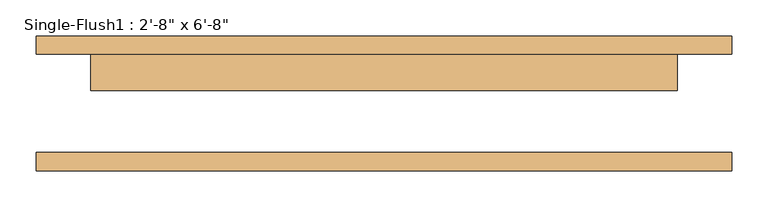
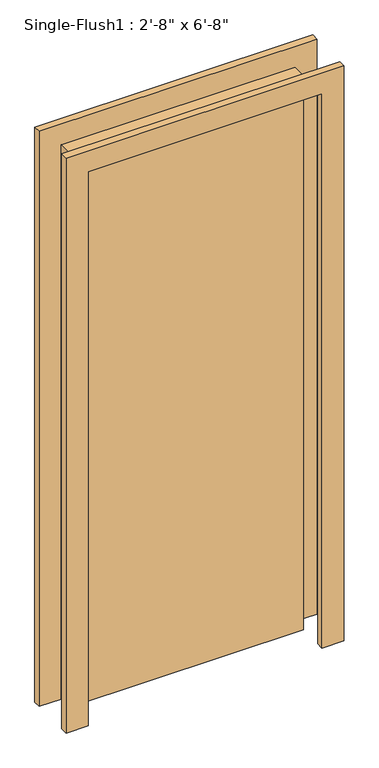
"""IFC4 building model written with IfcOpenShell, lengths in millimetres: door geometry."""

import ifcopenshell
import ifcopenshell.guid

model = None  # the IFC model being written
_history = None  # IfcOwnerHistory: only IFC2X3 demands one
_inside = {}  # id of a spatial element -> (the spatial element, [elements in it])
_under = {}  # id of a project, library or spatial element -> (it, [spatial elements below it])
_declared = {}  # id of a project -> (the project, [libraries it declares])
_typed = {}  # id of a type object -> (the type object, [elements of that type])
_made_of = {}  # id of a material, layer set ... -> (it, [elements and type objects made of it])


def new_model(schema):
    """Start an empty IFC model of exactly this schema.

    Asked for "IFC4X3", IfcOpenShell would pick the latest addendum, in which some entities
    have other attributes; the version numbers below select the first issue.
    IFC2X3 requires an IfcOwnerHistory on every rooted entity: one is made here for all.
    """
    global model, _history
    if schema == "IFC4X3":
        model = ifcopenshell.file(schema_version=(4, 3, 0, 0))
    else:
        model = ifcopenshell.file(schema=schema)
    _inside.clear()
    _under.clear()
    _declared.clear()
    _typed.clear()
    _made_of.clear()
    _history = None
    if model.schema == "IFC2X3":
        org = make("IfcOrganization", Name="unknown")
        user = make(
            "IfcPersonAndOrganization",
            ThePerson=make("IfcPerson", FamilyName="unknown"),
            TheOrganization=org,
        )
        app = make(
            "IfcApplication",
            ApplicationDeveloper=org,
            Version="unknown",
            ApplicationFullName="unknown",
            ApplicationIdentifier="unknown",
        )
        _history = make(
            "IfcOwnerHistory",
            OwningUser=user,
            OwningApplication=app,
            ChangeAction="ADDED",
            CreationDate=0,
        )
    return model


def make(cls, **values):
    """One entity of the class cls with the attributes given. An attribute that is None is left unset."""
    return model.create_entity(
        cls, **{name: value for name, value in values.items() if value is not None}
    )


def rooted(cls, **values):
    """An entity with a GlobalId (a new one), such as an element, a storey or a relation."""
    return make(cls, GlobalId=ifcopenshell.guid.new(), OwnerHistory=_history, **values)


def si_unit(unit_type, name, prefix=None):
    """IfcSIUnit, for example si_unit("LENGTHUNIT", "METRE", prefix="MILLI")."""
    return make("IfcSIUnit", UnitType=unit_type, Prefix=prefix, Name=name)


def assignment(units):
    """IfcUnitAssignment: the units of a project."""
    return None if units is None else make("IfcUnitAssignment", Units=units)


def point(xyz):
    """IfcCartesianPoint."""
    return None if xyz is None else make("IfcCartesianPoint", Coordinates=xyz)


def direction(xyz):
    """IfcDirection."""
    return None if xyz is None else make("IfcDirection", DirectionRatios=xyz)


def frame(location, z_axis=None, x_axis=None):
    """IfcAxis2Placement3D, a coordinate frame: its origin and axes. An axis left out is left unset."""
    return make(
        "IfcAxis2Placement3D",
        Location=point(location),
        Axis=direction(z_axis),
        RefDirection=direction(x_axis),
    )


def origin():
    """The frame at (0, 0, 0) with its axes left unset."""
    return frame((0.0, 0.0, 0.0))


def origin_with_axes():
    """The frame at (0, 0, 0) with the z axis (0, 0, 1) and the x axis (1, 0, 0) written out."""
    return frame((0.0, 0.0, 0.0), z_axis=(0.0, 0.0, 1.0), x_axis=(1.0, 0.0, 0.0))


def place(relative_to, where):
    """IfcLocalPlacement: puts the frame where relative to a parent placement (None: the world)."""
    return make(
        "IfcLocalPlacement", PlacementRelTo=relative_to, RelativePlacement=where
    )


def context(
    kind, dimensions, precision=None, world=None, true_north=None, identifier=None
):
    """IfcGeometricRepresentationContext, for example the 3D "Model" context."""
    return make(
        "IfcGeometricRepresentationContext",
        ContextIdentifier=identifier,
        ContextType=kind,
        CoordinateSpaceDimension=dimensions,
        Precision=precision,
        WorldCoordinateSystem=world,
        TrueNorth=true_north,
    )


def project(units=None, contexts=None):
    """IfcProject with its units and contexts."""
    return rooted(
        "IfcProject",
        Name="project",
        RepresentationContexts=contexts,
        UnitsInContext=assignment(units),
    )


def spatial(cls, under=None, at=None, **own):
    """A site, building, storey or space (cls), placed at a placement, below another one or the project."""
    s = rooted(cls, ObjectPlacement=at, **own)
    if under is not None:
        _under.setdefault(under.id(), (under, []))[1].append(s)
    return s


def polyline(points):
    """IfcPolyline through the points."""
    return make("IfcPolyline", Points=[point(p) for p in points])


def outline(outer, holes=None, kind="AREA"):
    """IfcArbitraryClosedProfileDef: a profile drawn as a closed curve; with holes, ...WithVoids."""
    if holes is None:
        return make("IfcArbitraryClosedProfileDef", ProfileType=kind, OuterCurve=outer)
    return make(
        "IfcArbitraryProfileDefWithVoids",
        ProfileType=kind,
        OuterCurve=outer,
        InnerCurves=holes,
    )


def extrude(swept, where, along, depth):
    """IfcExtrudedAreaSolid: the profile swept, set in the frame where, extruded along a direction by depth."""
    return make(
        "IfcExtrudedAreaSolid",
        SweptArea=swept,
        Position=where,
        ExtrudedDirection=direction(along),
        Depth=depth,
    )


def shape(context_of_items, identifier, shape_type, items):
    """IfcShapeRepresentation: the items that make up one representation, for example the "Body"."""
    return make(
        "IfcShapeRepresentation",
        ContextOfItems=context_of_items,
        RepresentationIdentifier=identifier,
        RepresentationType=shape_type,
        Items=items,
    )


def source(mapping_origin, context_of_items, identifier, shape_type, items):
    """IfcRepresentationMap: a shape defined once, which mapped items show again and again."""
    return make(
        "IfcRepresentationMap",
        MappingOrigin=mapping_origin,
        MappedRepresentation=shape(context_of_items, identifier, shape_type, items),
    )


def transform(
    local_origin,
    x_axis=None,
    y_axis=None,
    z_axis=None,
    scale=None,
    scale2=None,
    scale3=None,
    uniform=True,
):
    """IfcCartesianTransformationOperator3D, or its non-uniform kind. x_axis, y_axis, z_axis: its Axis1, 2, 3."""
    if uniform:
        return make(
            "IfcCartesianTransformationOperator3D",
            Axis1=direction(x_axis),
            Axis2=direction(y_axis),
            LocalOrigin=point(local_origin),
            Scale=scale,
            Axis3=direction(z_axis),
        )
    return make(
        "IfcCartesianTransformationOperator3DnonUniform",
        Axis1=direction(x_axis),
        Axis2=direction(y_axis),
        LocalOrigin=point(local_origin),
        Scale=scale,
        Axis3=direction(z_axis),
        Scale2=scale2,
        Scale3=scale3,
    )


def mapped(mapping_source, mapping_target):
    """IfcMappedItem: shows the shape of a source again, moved by a transform."""
    return make(
        "IfcMappedItem", MappingSource=mapping_source, MappingTarget=mapping_target
    )


def made_of(thing, what):
    """Note that an element or type object is made of a material, layer set ...; save() writes the relation."""
    if what is not None:
        _made_of.setdefault(what.id(), (what, []))[1].append(thing)
    return thing


def element(
    cls,
    number,
    at=None,
    inside=None,
    cuts=None,
    type_object=None,
    material=None,
    context=None,
    identifier="Body",
    shape_type=None,
    held_by="IfcProductDefinitionShape",
    body=None,
    shapes=None,
    **own,
):
    """One element of the class cls, such as IfcWall. Its Tag is "e" and its number.

    at: its placement. inside: the storey or other place that contains it. cuts: it is an
    opening in that element (IfcRelVoidsElement). A single representation is given by context,
    identifier, shape_type and body (its items); several are given by shapes. held_by: the class
    of the entity that holds the representations. save() writes the other relations.
    """
    e = rooted(cls, Tag="e%d" % number, ObjectPlacement=at, **own)
    if body is not None:
        shapes = [shape(context, identifier, shape_type, body)]
    if shapes is not None:
        e.Representation = make(held_by, Representations=shapes)
    if inside is not None:
        _inside.setdefault(inside.id(), (inside, []))[1].append(e)
    if cuts is not None:
        rooted(
            "IfcRelVoidsElement", RelatingBuildingElement=cuts, RelatedOpeningElement=e
        )
    if type_object is not None:
        _typed.setdefault(type_object.id(), (type_object, []))[1].append(e)
    return made_of(e, material)


def aggregate(whole, parts):
    """IfcRelAggregates: a whole, such as a stair, and the parts it consists of."""
    return rooted("IfcRelAggregates", RelatingObject=whole, RelatedObjects=parts)


def save(model, path):
    """Write the relations noted so far, then the file.

    IfcRelAggregates (storeys below a building ...), IfcRelContainedInSpatialStructure (elements
    in a storey), IfcRelDefinesByType, IfcRelAssociatesMaterial and IfcRelDeclares: one each for
    every whole, place, type object, material and project.
    """
    for whole, parts in _under.values():
        aggregate(whole, parts)
    for where, things in _inside.values():
        rooted(
            "IfcRelContainedInSpatialStructure",
            RelatedElements=things,
            RelatingStructure=where,
        )
    for kind, things in _typed.values():
        rooted("IfcRelDefinesByType", RelatedObjects=things, RelatingType=kind)
    for what, things in _made_of.values():
        rooted("IfcRelAssociatesMaterial", RelatedObjects=things, RelatingMaterial=what)
    for by, libraries in _declared.values():
        rooted("IfcRelDeclares", RelatingContext=by, RelatedDefinitions=libraries)
    model.write(path)


def door_2fa8c1c4(model_context):
    return source(origin(), model_context, "Body", "SweptSolid", [
        extrude(outline(polyline([(2108.2, -482.6), (0.0, -482.6), (0.0, -406.4), (2032.0, -406.4), (2032.0, 406.4), (0.0, 406.4), (0.0, 482.6), (2108.2, 482.6), (2108.2, -482.6)])), frame((0.0, 68.2625, 0.0), z_axis=(0.0, 1.0, 0.0), x_axis=(0.0, 0.0, 1.0)), (0.0, 0.0, 1.0), 25.4),
        extrude(outline(polyline([(2108.2, 482.6), (2108.2, -482.6), (0.0, -482.6), (0.0, -406.4), (2032.0, -406.4), (2032.0, 406.4), (0.0, 406.4), (0.0, 482.6), (2108.2, 482.6)])), frame((0.0, -93.6625, 0.0), z_axis=(0.0, 1.0, 0.0), x_axis=(0.0, 0.0, 1.0)), (0.0, 0.0, 1.0), 25.4),
        extrude(outline(polyline([(406.4, 17.4625), (-406.4, 17.4625), (-406.4, 68.2625), (406.4, 68.2625), (406.4, 17.4625)])), origin_with_axes(), (0.0, 0.0, 1.0), 2032.0),
    ])


if __name__ == "__main__":
    model = new_model("IFC4")
    model_context = context("Model", 3, world=origin())
    ifc_project = project(units=[si_unit("LENGTHUNIT", "METRE", prefix="MILLI")], contexts=[model_context])
    site = spatial("IfcSite", under=ifc_project)
    building = spatial("IfcBuilding", under=site)
    placement = place(None, origin())
    door_shape = door_2fa8c1c4(model_context)
    element("IfcDoor", 1, ObjectType="Single-Flush1 : 2'-8\" x 6'-8\"", at=placement, inside=building, context=model_context, shape_type="MappedRepresentation", body=[
        mapped(door_shape, transform((0.0, 0.0, 0.0), x_axis=(1.0, 0.0, 0.0), y_axis=(0.0, 1.0, 0.0), z_axis=(0.0, 0.0, 1.0))),
    ])
    save(model, "model.ifc")

# Revit data of these elements
# Type "Single-Flush1 : 2'-8\" x 6'-8\""
#   Type Mark = "23"
#   Construction Type Id = "MDOOR"
#   Assembly Code = "C1020"
#   Analytic Construction = "Metal"
#   Thickness = 0' - 2"
#   Heat Transfer Coefficient (U) = 3.7021 W/(m²·K)
#   Height = 6' - 8"
#   Trim Projection Ext = 0' - 1"
#   Trim Projection Int = 0' - 1"
#   Trim Width = 0' - 3"
#   Width = 2' - 8"
#   Door Material = Door - Panel
#   Frame Material = Door - Frame
#   Visual Light Transmittance = 0
#   Solar Heat Gain Coefficient = 0
#   Function = (empty or 0)
#   Wall Closure = (empty or 0)
# Element 1 (IfcDoor, "Single-Flush1 : 2'-8\" x 6'-8\"")
#   Materials on its faces: "Door - Frame", "Door - Panel"
# Materials
#   "Door - Panel": class "Wood", colour RGB 210 159 95, transparency 0, Cost = 0
#   "Door - Frame": class "Miscellaneous", colour RGB 118 70 51, transparency 0, Cost = 0
